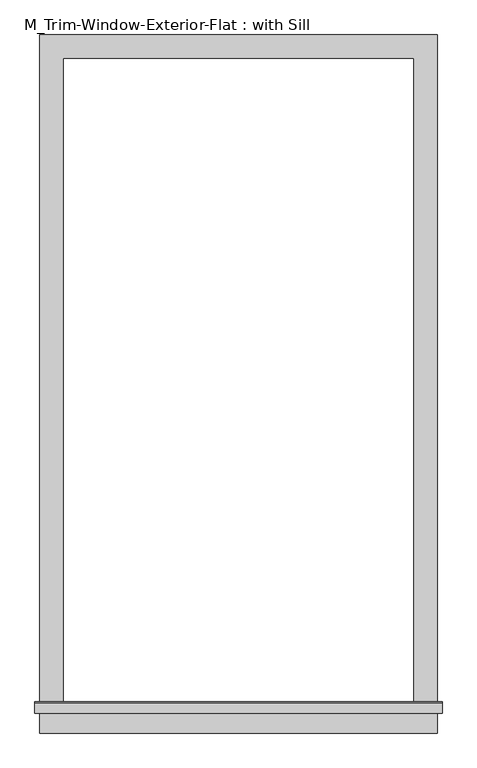
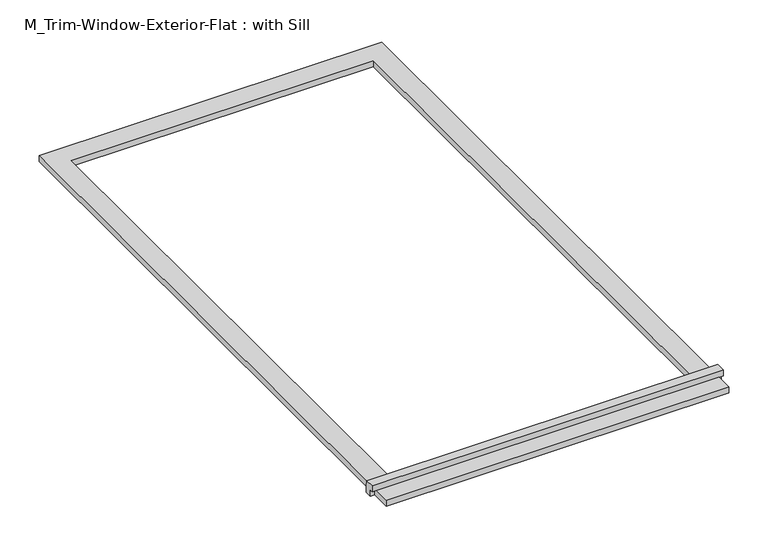
"""IFC4 building model written with IfcOpenShell, lengths in millimetres: proxy geometry, M_Trim-Window-Exterior-Flat : with Sill."""

from ifc_helpers import new_model, si_unit, frame, origin, origin_with_axes, place, context, project, spatial, polyline, outline, extrude, source, transform, mapped, element, save


def m_trim_window_exterior_flat_with_sill_09d1e46a(model_context):
    return source(origin(), model_context, "Body", "SweptSolid", [
        extrude(outline(polyline([(510.0, -1670.4323709), (510.0, -1730.4323709), (-510.0, -1730.4323709), (-510.0, -1670.4323709), (510.0, -1670.4323709)])), origin_with_axes(), (0.0, 0.0, 1.0), 19.05),
        extrude(outline(polyline([(-1680.0, 38.1), (-1652.4580645, 38.1), (-1650.0, 19.05), (-1650.0, 0.0), (-1670.4323709, 0.0), (-1670.4323709, 19.05), (-1680.0, 19.05), (-1680.0, 38.1)])), frame((-522.7, 0.0, 0.0), z_axis=(1.0, 0.0, 0.0), x_axis=(0.0, 1.0, 0.0)), (0.0, 0.0, 1.0), 1045.4),
        extrude(outline(polyline([(-510.0, 60.0), (510.0, 60.0), (510.0, -1650.0), (450.0, -1650.0), (450.0, 0.0), (-450.0, 0.0), (-450.0, -1650.0), (-510.0, -1650.0), (-510.0, 60.0)])), origin_with_axes(), (0.0, 0.0, 1.0), 19.05),
    ])


if __name__ == "__main__":
    model = new_model("IFC4")
    model_context = context("Model", 3, world=origin())
    ifc_project = project(units=[si_unit("LENGTHUNIT", "METRE", prefix="MILLI")], contexts=[model_context])
    site = spatial("IfcSite", under=ifc_project)
    building = spatial("IfcBuilding", under=site)
    placement = place(None, origin())
    m_trim_window_exterior_flat_with_sill_shape = m_trim_window_exterior_flat_with_sill_09d1e46a(model_context)
    element("IfcBuildingElementProxy", 1, Name="M_Trim-Window-Exterior-Flat : with Sill", ObjectType="M_Trim-Window-Exterior-Flat : with Sill", at=placement, inside=building, context=model_context, shape_type="MappedRepresentation", body=[
        mapped(m_trim_window_exterior_flat_with_sill_shape, transform((0.0, 0.0, 0.0), x_axis=(1.0, 0.0, 0.0), y_axis=(0.0, 1.0, 0.0), z_axis=(0.0, 0.0, 1.0))),
    ])
    save(model, "model.ifc")

# Revit data of these elements
# Project information
#   Organization Name = "Organization Name"
#   Organization Description = "Organization Description"
#   Building Name = "Building Name"
#   Project Issue Date = "Issue Date"
#   Project Status = "Project Status"
#   Client Name = "Client Name"
#   Project Address = "Enter address here\nAddress Line 2"
#   Project Name = "Project Name"
#   Project Number = "Project Number"
# Type "M_Trim-Window-Exterior-Flat : with Sill"
#   Trim Width = 60 mm
#   Trim Thickness_Picture Frame = 30 mm
#   Trim Thickness_with Sill = 19.05 mm
#   Sill Thickness = 30 mm
#   Opening Width [instance default] = 600 mm
#   Opening Height [instance default] = 900 mm
#   Default Elevation = 1200 mm
#   Sill = yes
#   Picture Frame = no
#   Trim Material [instance default] = none
# Element 1 (IfcBuildingElementProxy, "M_Trim-Window-Exterior-Flat : with Sill")
#   Opening Width = 900 mm
#   Opening Height = 1650 mm
#   Trim Material = Clad - White
#   Materials on its faces: "Clad - White"
# Materials
#   "Clad - White": class "Wood", colour RGB 245 245 243, transparency 0, Cost = 0
